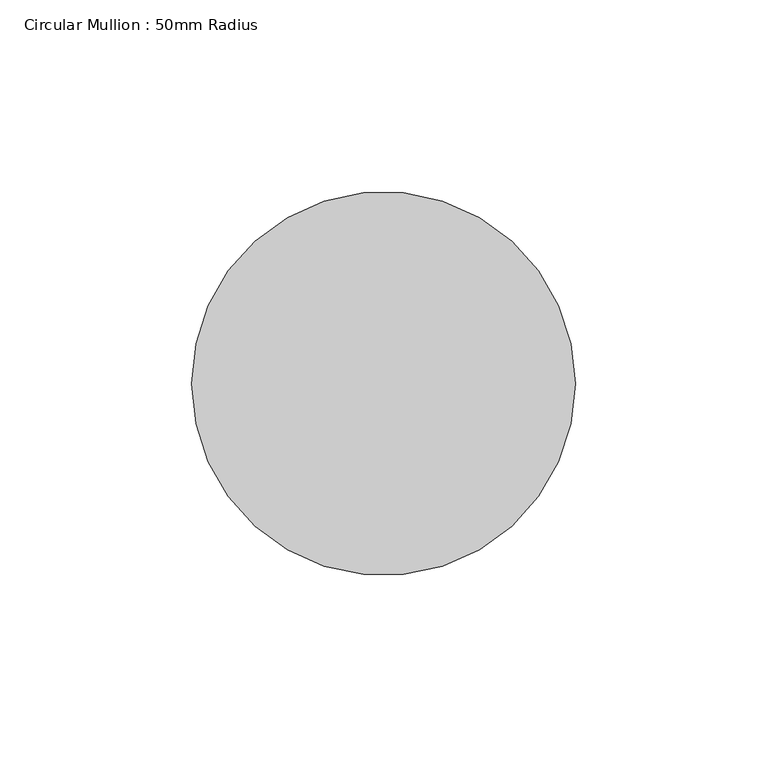
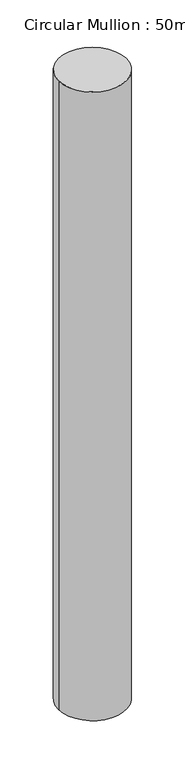
"""IFC4 building model written with IfcOpenShell, lengths in millimetres: member geometry, Circular Mullion : 50mm Radius."""

from ifc_helpers import new_model, si_unit, point, frame, origin, origin_2d, place, context, project, spatial, circle_curve, trimmed, segment, composite_curve, outline, extrude, source, transform, mapped, element, save


def circular_mullion_50mm_radius_11e91cbb(model_context):
    return source(origin(), model_context, "Body", "SweptSolid", [
        extrude(outline(composite_curve([segment(trimmed(circle_curve(origin_2d(), 50.0), [point((50.0, 0.0))], [point((-50.0, 0.0))], False, "CARTESIAN"), True, "CONTINUOUS"), segment(trimmed(circle_curve(origin_2d(), 50.0), [point((-50.0, 0.0))], [point((50.0, 0.0))], False, "CARTESIAN"), True, "CONTINUOUS")], self_intersect=False)), frame((0.0, 0.0, -982.7759642), z_axis=(0.0, 0.0, 1.0), x_axis=(1.0, 0.0, 0.0)), (0.0, 0.0, 1.0), 982.7759642),
    ])


if __name__ == "__main__":
    model = new_model("IFC4")
    model_context = context("Model", 3, world=origin())
    ifc_project = project(units=[si_unit("LENGTHUNIT", "METRE", prefix="MILLI")], contexts=[model_context])
    site = spatial("IfcSite", under=ifc_project)
    building = spatial("IfcBuilding", under=site)
    placement = place(None, origin())
    circular_mullion_50mm_radius_shape = circular_mullion_50mm_radius_11e91cbb(model_context)
    element("IfcMember", 1, ObjectType="Circular Mullion : 50mm Radius", at=placement, inside=building, context=model_context, shape_type="MappedRepresentation", body=[
        mapped(circular_mullion_50mm_radius_shape, transform((0.0, 0.0, 0.0), x_axis=(1.0, 0.0, 0.0), y_axis=(0.0, 1.0, 0.0), z_axis=(0.0, 0.0, 1.0))),
    ])
    save(model, "model.ifc")

# Revit data of these elements
# Type "Circular Mullion : 50mm Radius"
#   built-in parameter 1007350 = 0.164042 (stored number, unit not read)
# Element 1 (IfcMember, "Circular Mullion : 50mm Radius")
#   Materials on its faces: "Aluminium"
# Materials
#   "Aluminium": class "Metal", colour RGB 247 247 247, transparency 0, Description = "Aluminium 6061", Cost = 0
